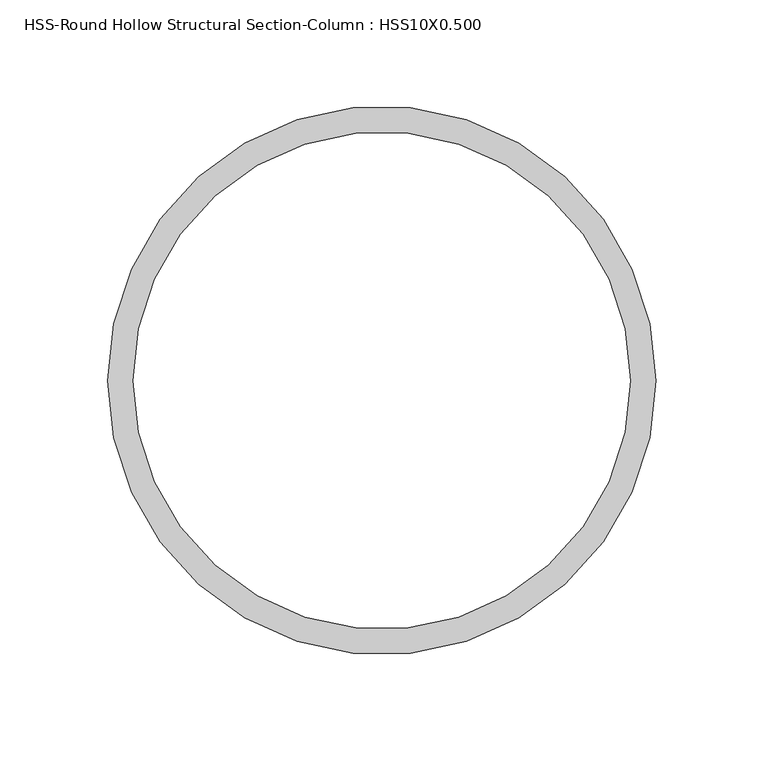
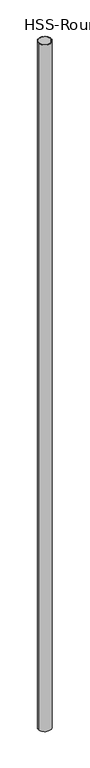
"""IFC4 building model written with IfcOpenShell, lengths in millimetres: column geometry, HSS-Round Hollow Structural Section-Column : HSS10X0.500."""

import ifcopenshell
import ifcopenshell.guid

model = None  # the IFC model being written
_history = None  # IfcOwnerHistory: only IFC2X3 demands one
_inside = {}  # id of a spatial element -> (the spatial element, [elements in it])
_under = {}  # id of a project, library or spatial element -> (it, [spatial elements below it])
_declared = {}  # id of a project -> (the project, [libraries it declares])
_typed = {}  # id of a type object -> (the type object, [elements of that type])
_made_of = {}  # id of a material, layer set ... -> (it, [elements and type objects made of it])


def new_model(schema):
    """Start an empty IFC model of exactly this schema.

    Asked for "IFC4X3", IfcOpenShell would pick the latest addendum, in which some entities
    have other attributes; the version numbers below select the first issue.
    IFC2X3 requires an IfcOwnerHistory on every rooted entity: one is made here for all.
    """
    global model, _history
    if schema == "IFC4X3":
        model = ifcopenshell.file(schema_version=(4, 3, 0, 0))
    else:
        model = ifcopenshell.file(schema=schema)
    _inside.clear()
    _under.clear()
    _declared.clear()
    _typed.clear()
    _made_of.clear()
    _history = None
    if model.schema == "IFC2X3":
        org = make("IfcOrganization", Name="unknown")
        user = make(
            "IfcPersonAndOrganization",
            ThePerson=make("IfcPerson", FamilyName="unknown"),
            TheOrganization=org,
        )
        app = make(
            "IfcApplication",
            ApplicationDeveloper=org,
            Version="unknown",
            ApplicationFullName="unknown",
            ApplicationIdentifier="unknown",
        )
        _history = make(
            "IfcOwnerHistory",
            OwningUser=user,
            OwningApplication=app,
            ChangeAction="ADDED",
            CreationDate=0,
        )
    return model


def make(cls, **values):
    """One entity of the class cls with the attributes given. An attribute that is None is left unset."""
    return model.create_entity(
        cls, **{name: value for name, value in values.items() if value is not None}
    )


def rooted(cls, **values):
    """An entity with a GlobalId (a new one), such as an element, a storey or a relation."""
    return make(cls, GlobalId=ifcopenshell.guid.new(), OwnerHistory=_history, **values)


def si_unit(unit_type, name, prefix=None):
    """IfcSIUnit, for example si_unit("LENGTHUNIT", "METRE", prefix="MILLI")."""
    return make("IfcSIUnit", UnitType=unit_type, Prefix=prefix, Name=name)


def assignment(units):
    """IfcUnitAssignment: the units of a project."""
    return None if units is None else make("IfcUnitAssignment", Units=units)


def point(xyz):
    """IfcCartesianPoint."""
    return None if xyz is None else make("IfcCartesianPoint", Coordinates=xyz)


def direction(xyz):
    """IfcDirection."""
    return None if xyz is None else make("IfcDirection", DirectionRatios=xyz)


def frame(location, z_axis=None, x_axis=None):
    """IfcAxis2Placement3D, a coordinate frame: its origin and axes. An axis left out is left unset."""
    return make(
        "IfcAxis2Placement3D",
        Location=point(location),
        Axis=direction(z_axis),
        RefDirection=direction(x_axis),
    )


def frame_2d(location, x_axis=None):
    """IfcAxis2Placement2D, a coordinate frame in the plane: its origin and x axis."""
    return make(
        "IfcAxis2Placement2D", Location=point(location), RefDirection=direction(x_axis)
    )


def origin():
    """The frame at (0, 0, 0) with its axes left unset."""
    return frame((0.0, 0.0, 0.0))


def origin_2d():
    """The frame at (0, 0) in the plane with its x axis left unset."""
    return frame_2d((0.0, 0.0))


def place(relative_to, where):
    """IfcLocalPlacement: puts the frame where relative to a parent placement (None: the world)."""
    return make(
        "IfcLocalPlacement", PlacementRelTo=relative_to, RelativePlacement=where
    )


def context(
    kind, dimensions, precision=None, world=None, true_north=None, identifier=None
):
    """IfcGeometricRepresentationContext, for example the 3D "Model" context."""
    return make(
        "IfcGeometricRepresentationContext",
        ContextIdentifier=identifier,
        ContextType=kind,
        CoordinateSpaceDimension=dimensions,
        Precision=precision,
        WorldCoordinateSystem=world,
        TrueNorth=true_north,
    )


def project(units=None, contexts=None):
    """IfcProject with its units and contexts."""
    return rooted(
        "IfcProject",
        Name="project",
        RepresentationContexts=contexts,
        UnitsInContext=assignment(units),
    )


def spatial(cls, under=None, at=None, **own):
    """A site, building, storey or space (cls), placed at a placement, below another one or the project."""
    s = rooted(cls, ObjectPlacement=at, **own)
    if under is not None:
        _under.setdefault(under.id(), (under, []))[1].append(s)
    return s


def circle_curve(where, radius):
    """IfcCircle in the frame where."""
    return make("IfcCircle", Position=where, Radius=radius)


def trimmed(basis, trim1, trim2, sense, master):
    """IfcTrimmedCurve: the piece of a basis curve between two trims."""
    return make(
        "IfcTrimmedCurve",
        BasisCurve=basis,
        Trim1=trim1,
        Trim2=trim2,
        SenseAgreement=sense,
        MasterRepresentation=master,
    )


def segment(curve, same_sense, transition):
    """IfcCompositeCurveSegment."""
    return make(
        "IfcCompositeCurveSegment",
        Transition=transition,
        SameSense=same_sense,
        ParentCurve=curve,
    )


def composite_curve(segments, self_intersect=None):
    """IfcCompositeCurve: segments joined end to end."""
    return make("IfcCompositeCurve", Segments=segments, SelfIntersect=self_intersect)


def outline(outer, holes=None, kind="AREA"):
    """IfcArbitraryClosedProfileDef: a profile drawn as a closed curve; with holes, ...WithVoids."""
    if holes is None:
        return make("IfcArbitraryClosedProfileDef", ProfileType=kind, OuterCurve=outer)
    return make(
        "IfcArbitraryProfileDefWithVoids",
        ProfileType=kind,
        OuterCurve=outer,
        InnerCurves=holes,
    )


def extrude(swept, where, along, depth):
    """IfcExtrudedAreaSolid: the profile swept, set in the frame where, extruded along a direction by depth."""
    return make(
        "IfcExtrudedAreaSolid",
        SweptArea=swept,
        Position=where,
        ExtrudedDirection=direction(along),
        Depth=depth,
    )


def shape(context_of_items, identifier, shape_type, items):
    """IfcShapeRepresentation: the items that make up one representation, for example the "Body"."""
    return make(
        "IfcShapeRepresentation",
        ContextOfItems=context_of_items,
        RepresentationIdentifier=identifier,
        RepresentationType=shape_type,
        Items=items,
    )


def source(mapping_origin, context_of_items, identifier, shape_type, items):
    """IfcRepresentationMap: a shape defined once, which mapped items show again and again."""
    return make(
        "IfcRepresentationMap",
        MappingOrigin=mapping_origin,
        MappedRepresentation=shape(context_of_items, identifier, shape_type, items),
    )


def transform(
    local_origin,
    x_axis=None,
    y_axis=None,
    z_axis=None,
    scale=None,
    scale2=None,
    scale3=None,
    uniform=True,
):
    """IfcCartesianTransformationOperator3D, or its non-uniform kind. x_axis, y_axis, z_axis: its Axis1, 2, 3."""
    if uniform:
        return make(
            "IfcCartesianTransformationOperator3D",
            Axis1=direction(x_axis),
            Axis2=direction(y_axis),
            LocalOrigin=point(local_origin),
            Scale=scale,
            Axis3=direction(z_axis),
        )
    return make(
        "IfcCartesianTransformationOperator3DnonUniform",
        Axis1=direction(x_axis),
        Axis2=direction(y_axis),
        LocalOrigin=point(local_origin),
        Scale=scale,
        Axis3=direction(z_axis),
        Scale2=scale2,
        Scale3=scale3,
    )


def mapped(mapping_source, mapping_target):
    """IfcMappedItem: shows the shape of a source again, moved by a transform."""
    return make(
        "IfcMappedItem", MappingSource=mapping_source, MappingTarget=mapping_target
    )


def made_of(thing, what):
    """Note that an element or type object is made of a material, layer set ...; save() writes the relation."""
    if what is not None:
        _made_of.setdefault(what.id(), (what, []))[1].append(thing)
    return thing


def element(
    cls,
    number,
    at=None,
    inside=None,
    cuts=None,
    type_object=None,
    material=None,
    context=None,
    identifier="Body",
    shape_type=None,
    held_by="IfcProductDefinitionShape",
    body=None,
    shapes=None,
    **own,
):
    """One element of the class cls, such as IfcWall. Its Tag is "e" and its number.

    at: its placement. inside: the storey or other place that contains it. cuts: it is an
    opening in that element (IfcRelVoidsElement). A single representation is given by context,
    identifier, shape_type and body (its items); several are given by shapes. held_by: the class
    of the entity that holds the representations. save() writes the other relations.
    """
    e = rooted(cls, Tag="e%d" % number, ObjectPlacement=at, **own)
    if body is not None:
        shapes = [shape(context, identifier, shape_type, body)]
    if shapes is not None:
        e.Representation = make(held_by, Representations=shapes)
    if inside is not None:
        _inside.setdefault(inside.id(), (inside, []))[1].append(e)
    if cuts is not None:
        rooted(
            "IfcRelVoidsElement", RelatingBuildingElement=cuts, RelatedOpeningElement=e
        )
    if type_object is not None:
        _typed.setdefault(type_object.id(), (type_object, []))[1].append(e)
    return made_of(e, material)


def aggregate(whole, parts):
    """IfcRelAggregates: a whole, such as a stair, and the parts it consists of."""
    return rooted("IfcRelAggregates", RelatingObject=whole, RelatedObjects=parts)


def save(model, path):
    """Write the relations noted so far, then the file.

    IfcRelAggregates (storeys below a building ...), IfcRelContainedInSpatialStructure (elements
    in a storey), IfcRelDefinesByType, IfcRelAssociatesMaterial and IfcRelDeclares: one each for
    every whole, place, type object, material and project.
    """
    for whole, parts in _under.values():
        aggregate(whole, parts)
    for where, things in _inside.values():
        rooted(
            "IfcRelContainedInSpatialStructure",
            RelatedElements=things,
            RelatingStructure=where,
        )
    for kind, things in _typed.values():
        rooted("IfcRelDefinesByType", RelatedObjects=things, RelatingType=kind)
    for what, things in _made_of.values():
        rooted("IfcRelAssociatesMaterial", RelatedObjects=things, RelatingMaterial=what)
    for by, libraries in _declared.values():
        rooted("IfcRelDeclares", RelatingContext=by, RelatedDefinitions=libraries)
    model.write(path)


def hss_round_hollow_structural_section_column_hss10x0_500_9719e917(model_context):
    return source(origin(), model_context, "Body", "SweptSolid", [
        extrude(outline(composite_curve([segment(trimmed(circle_curve(origin_2d(), 127.0), [point((-127.0, 0.0))], [point((127.0, 0.0))], False, "CARTESIAN"), True, "CONTINUOUS"), segment(trimmed(circle_curve(origin_2d(), 127.0), [point((127.0, 0.0))], [point((-127.0, 0.0))], False, "CARTESIAN"), True, "CONTINUOUS")], self_intersect=False), holes=[composite_curve([segment(trimmed(circle_curve(origin_2d(), 115.189), [point((-115.189, 0.0))], [point((115.189, 0.0))], True, "CARTESIAN"), True, "CONTINUOUS"), segment(trimmed(circle_curve(origin_2d(), 115.189), [point((115.189, 0.0))], [point((-115.189, 0.0))], True, "CARTESIAN"), True, "CONTINUOUS")], self_intersect=False)]), frame((0.0, 0.0, 5969.0), z_axis=(0.0, 0.0, 1.0), x_axis=(1.0, 0.0, 0.0)), (0.0, 0.0, 1.0), 14376.4),
    ])


if __name__ == "__main__":
    model = new_model("IFC4")
    model_context = context("Model", 3, world=origin())
    ifc_project = project(units=[si_unit("LENGTHUNIT", "METRE", prefix="MILLI")], contexts=[model_context])
    site = spatial("IfcSite", under=ifc_project)
    building = spatial("IfcBuilding", under=site)
    placement = place(None, origin())
    hss_round_hollow_structural_section_column_hss10x0_500_shape = hss_round_hollow_structural_section_column_hss10x0_500_9719e917(model_context)
    element("IfcColumn", 1, ObjectType="HSS-Round Hollow Structural Section-Column : HSS10X0.500", at=placement, inside=building, context=model_context, shape_type="MappedRepresentation", body=[
        mapped(hss_round_hollow_structural_section_column_hss10x0_500_shape, transform((0.0, 0.0, 0.0), x_axis=(1.0, 0.0, 0.0), y_axis=(0.0, 1.0, 0.0), z_axis=(0.0, 0.0, 1.0))),
    ])
    save(model, "model.ifc")

# Revit data of these elements
# Type "HSS-Round Hollow Structural Section-Column : HSS10X0.500"
#   Assembly Code = "B10"
#   W = 50.8
#   OD = 0' - 10"
#   t = 0' - 0.465"
#   A = 0.0965278 SF
#   Column Material [instance default] = Metal - Steel - ASTM A53
# Element 1 (IfcColumn, "HSS-Round Hollow Structural Section-Column : HSS10X0.500")
#   Materials on its faces: "Metal - Steel - ASTM A53"
# Materials
#   "Metal - Steel - ASTM A53": class "Metal", colour RGB 128 0 0, transparency 0
